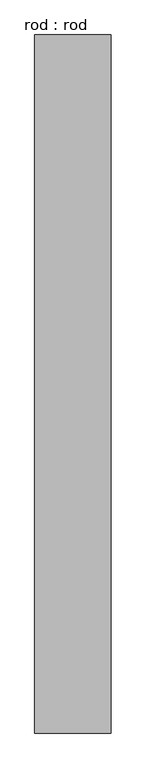
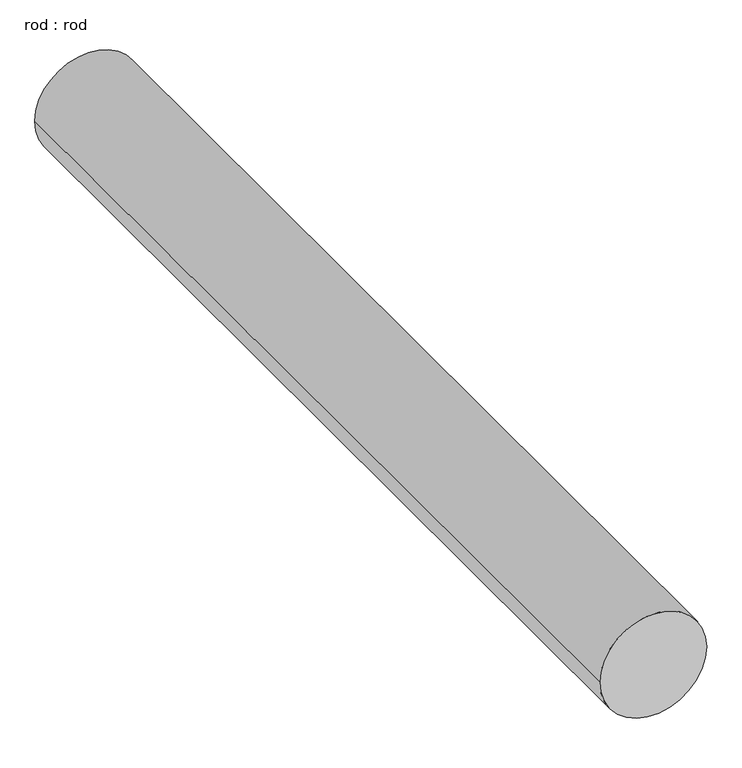
"""IFC4 building model written with IfcOpenShell, lengths in millimetres: proxy geometry, rod : rod."""

from ifc_helpers import new_model, si_unit, point, frame, frame_2d, origin, place, context, project, spatial, circle_curve, trimmed, segment, composite_curve, outline, extrude, source, transform, mapped, element, save


def rod_rod_19028cf9(model_context):
    return source(origin(), model_context, "Body", "SweptSolid", [
        extrude(outline(composite_curve([segment(trimmed(circle_curve(frame_2d((0.0108462, 0.0)), 200.0), [point((0.0108462, 200.0))], [point((0.0108462, -200.0))], False, "CARTESIAN"), True, "CONTINUOUS"), segment(trimmed(circle_curve(frame_2d((0.0108462, 0.0)), 200.0), [point((0.0108462, -200.0))], [point((0.0108462, 200.0))], False, "CARTESIAN"), True, "CONTINUOUS")], self_intersect=False)), frame((0.0, 2265.1191795, 0.0), z_axis=(0.0, 1.0, 0.0), x_axis=(0.0, 0.0, 1.0)), (0.0, 0.0, 1.0), 3655.2188717),
    ])


if __name__ == "__main__":
    model = new_model("IFC4")
    model_context = context("Model", 3, world=origin())
    ifc_project = project(units=[si_unit("LENGTHUNIT", "METRE", prefix="MILLI")], contexts=[model_context])
    site = spatial("IfcSite", under=ifc_project)
    building = spatial("IfcBuilding", under=site)
    placement = place(None, origin())
    rod_rod_shape = rod_rod_19028cf9(model_context)
    element("IfcBuildingElementProxy", 1, Name="rod : rod", ObjectType="rod : rod", at=placement, inside=building, context=model_context, shape_type="MappedRepresentation", body=[
        mapped(rod_rod_shape, transform((0.0, 0.0, 0.0), x_axis=(1.0, 0.0, 0.0), y_axis=(0.0, 1.0, 0.0), z_axis=(0.0, 0.0, 1.0))),
    ])
    save(model, "model.ifc")

# Revit data of these elements
# Type "rod : rod"
#   Default Elevation = 0
